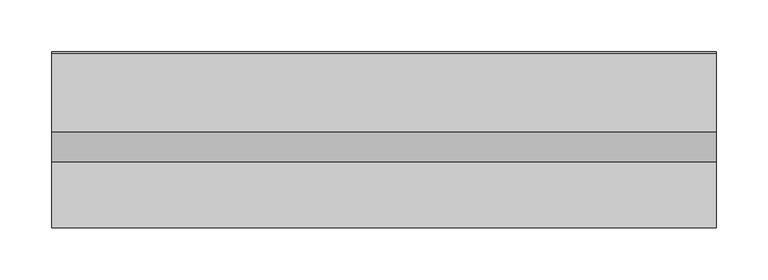
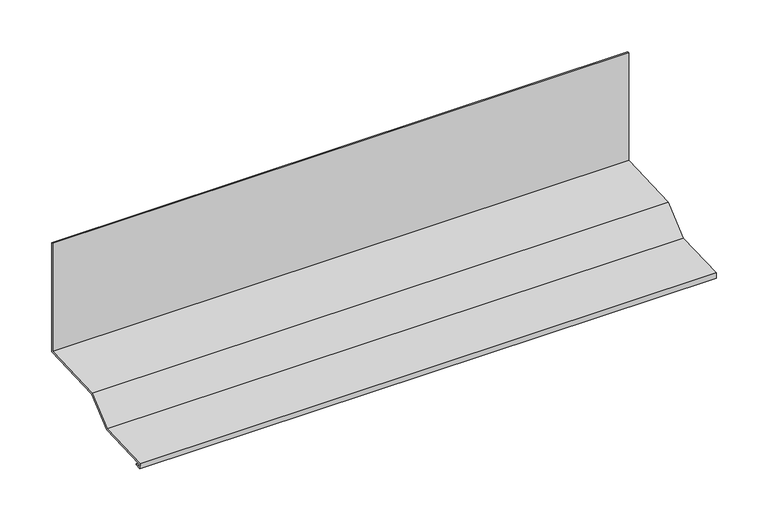
"""IFC4 building model written with IfcOpenShell, lengths in millimetres: proxy geometry, Generic Models 7:Generic Models 1:337419:Generic Models 1:337419 : Generic Models 7:Generic Models 1:337419:49 : Generic Models 7:Generic Models 1:337419:Generic Models 1:337419 : Generic Models 7:Generic Models 1:337419:301336."""

from ifc_helpers import new_model, si_unit, frame, origin, place, context, project, spatial, polyline, outline, extrude, source, transform, mapped, element, save


def generic_models_1eaec0d2(model_context):
    return source(origin(), model_context, "Body", "SweptSolid", [
        extrude(outline(polyline([(-579014.9788841, 4044.5784977), (-579014.9788841, 4171.5784977), (-579013.3913841, 4171.5784977), (-579013.3913841, 4043.0557661), (-579090.5065581, 4039.8426339), (-579119.6928514, 4015.352426), (-579182.0918554, 4012.7524675), (-579181.9596785, 4009.58022), (-579176.2031328, 4009.820076), (-579176.2031328, 4008.2311986), (-579183.4797137, 4007.9280077), (-579183.7440677, 4014.2725027), (-579120.2991176, 4016.9160423), (-579091.1128243, 4041.4062502), (-579014.9788841, 4044.5784977)])), frame((578741.5428078, 0.0, 0.0), z_axis=(1.0, 0.0, 0.0), x_axis=(0.0, 1.0, 0.0)), (0.0, 0.0, 1.0), 642.3689161),
    ])


if __name__ == "__main__":
    model = new_model("IFC4")
    model_context = context("Model", 3, world=origin())
    ifc_project = project(units=[si_unit("LENGTHUNIT", "METRE", prefix="MILLI")], contexts=[model_context])
    site = spatial("IfcSite", under=ifc_project)
    building = spatial("IfcBuilding", under=site)
    placement = place(None, origin())
    generic_models_shape = generic_models_1eaec0d2(model_context)
    element("IfcBuildingElementProxy", 1, Name="Generic Models 7:Generic Models 1:337419:Generic Models 1:337419 : Generic Models 7:Generic Models 1:337419:49 : Generic Models 7:Generic Models 1:337419:Generic Models 1:337419 : Generic Models 7:Generic Models 1:337419:301336", ObjectType="Generic Models 7:Generic Models 1:337419:Generic Models 1:337419 : Generic Models 7:Generic Models 1:337419:49 : Generic Models 7:Generic Models 1:337419:Generic Models 1:337419 : Generic Models 7:Generic Models 1:337419:301336", at=placement, inside=building, context=model_context, shape_type="MappedRepresentation", body=[
        mapped(generic_models_shape, transform((0.0, 0.0, 0.0), x_axis=(1.0, 0.0, 0.0), y_axis=(0.0, 1.0, 0.0), z_axis=(0.0, 0.0, 1.0))),
    ])
    save(model, "model.ifc")

# Revit data of these elements
# Type "Generic Models 7:Generic Models 1:337419:Generic Models 1:337419 : Generic Models 7:Generic Models 1:337419:49 : Generic Models 7:Generic Models 1:337419:Generic Models 1:337419 : Generic Models 7:Generic Models 1:337419:301336"
#   NameOverride = "Generic Models 7:Generic Models 1:337419:Generic Models 1:337419 : Generic Models 7:Generic Models 1:337419:301336"
#   ObjectTypeOverride = "Generic Models 1:337419 : Generic Models 7:Generic Models 1:337419"
#   Reference = "Generic Models 1"
#   Tag = "301336"
# Element 1 (IfcBuildingElementProxy, "Generic Models 7:Generic Models 1:337419:Generic Models 1:337419 : Generic Models 7:Generic Models 1:337419:49 : Generic Models 7:Generic Models 1:337419:Generic Models 1:337419 : Generic Models 7:Generic Models 1:337419:301336")
#   Materials on its faces: "PARAPET HIGH EAVE TRIM"
# Materials
#   "PARAPET HIGH EAVE TRIM": class "Unassigned", colour RGB 182 182 182, transparency 0, Cost = 0
